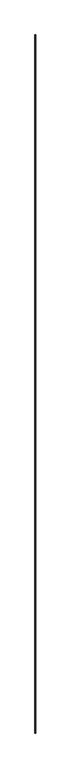
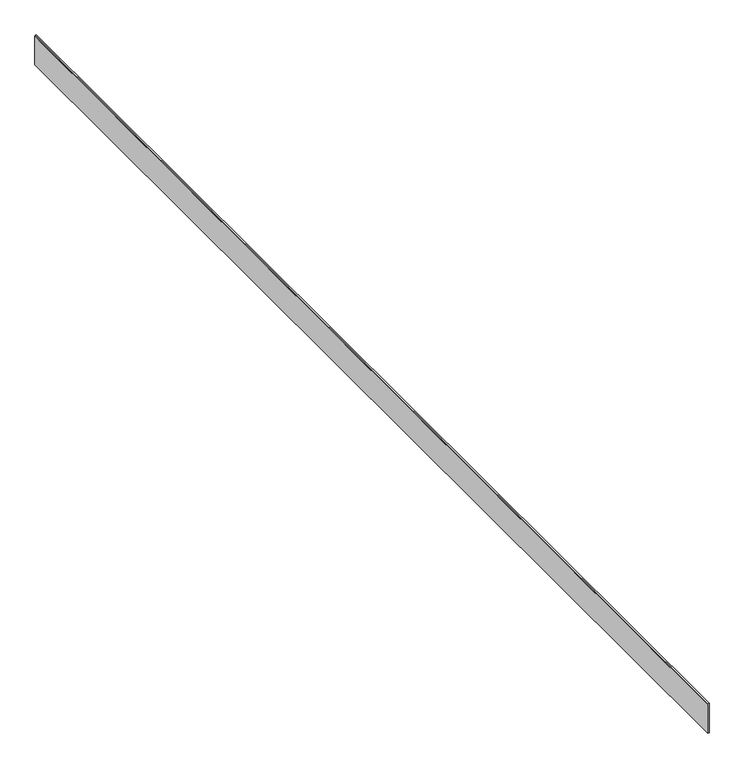
"""IFC4 building model written with IfcOpenShell, lengths in millimetres: proxy geometry, Generic Models 7:Generic Models 1:6:Generic Models 1:6 : Generic Models 7:Generic Models 1:337419:11 : Generic Models 7:Generic Models 1:6:Generic Models 1:6 : Generic Models 7:Generic Models 1:337419:312901."""

from ifc_helpers import new_model, si_unit, frame, origin, place, context, project, spatial, polyline, outline, extrude, source, transform, mapped, element, save


def generic_models_ca5898e6(model_context):
    return source(origin(), model_context, "Body", "SweptSolid", [
        extrude(outline(polyline([(-80.922555, 667585.4117239), (-1222.375, 667585.4117239), (-1222.375, 667636.2117239), (-37.30625, 667636.2117239), (-37.30625, 667593.3180904), (-80.922555, 667593.3180904), (-80.922555, 667585.4117239)])), frame((0.0, -578051.3663841, 0.0), z_axis=(0.0, 1.0, 0.0), x_axis=(0.0, 0.0, 1.0)), (0.0, 0.0, 1.0), 44500.8),
    ])


if __name__ == "__main__":
    model = new_model("IFC4")
    model_context = context("Model", 3, world=origin())
    ifc_project = project(units=[si_unit("LENGTHUNIT", "METRE", prefix="MILLI")], contexts=[model_context])
    site = spatial("IfcSite", under=ifc_project)
    building = spatial("IfcBuilding", under=site)
    placement = place(None, origin())
    generic_models_shape = generic_models_ca5898e6(model_context)
    element("IfcBuildingElementProxy", 1, Name="Generic Models 7:Generic Models 1:6:Generic Models 1:6 : Generic Models 7:Generic Models 1:337419:11 : Generic Models 7:Generic Models 1:6:Generic Models 1:6 : Generic Models 7:Generic Models 1:337419:312901", ObjectType="Generic Models 7:Generic Models 1:6:Generic Models 1:6 : Generic Models 7:Generic Models 1:337419:11 : Generic Models 7:Generic Models 1:6:Generic Models 1:6 : Generic Models 7:Generic Models 1:337419:312901", at=placement, inside=building, context=model_context, shape_type="MappedRepresentation", body=[
        mapped(generic_models_shape, transform((0.0, 0.0, 0.0), x_axis=(1.0, 0.0, 0.0), y_axis=(0.0, 1.0, 0.0), z_axis=(0.0, 0.0, 1.0))),
    ])
    save(model, "model.ifc")

# Revit data of these elements
# Type "Generic Models 7:Generic Models 1:6:Generic Models 1:6 : Generic Models 7:Generic Models 1:337419:11 : Generic Models 7:Generic Models 1:6:Generic Models 1:6 : Generic Models 7:Generic Models 1:337419:312901"
#   NameOverride = "Generic Models 7:Generic Models 1:6:Generic Models 1:6 : Generic Models 7:Generic Models 1:337419:312901"
#   ObjectTypeOverride = "Generic Models 1:6 : Generic Models 7:Generic Models 1:337419"
#   Reference = "Generic Models 1"
#   Tag = "312901"
# Element 1 (IfcBuildingElementProxy, "Generic Models 7:Generic Models 1:6:Generic Models 1:6 : Generic Models 7:Generic Models 1:337419:11 : Generic Models 7:Generic Models 1:6:Generic Models 1:6 : Generic Models 7:Generic Models 1:337419:312901")
#   Materials on its faces: "EXTRUDED POLYSTYRENE (XPS) RIGID FOAM INSULATION (FOAMULAR® 250 OR SIMILAR)"
# Materials
#   "EXTRUDED POLYSTYRENE (XPS) RIGID FOAM INSULATION (FOAMULAR® 250 OR SIMILAR)": class "Unassigned", colour RGB 247 185 194, transparency 0, Cost = 0
